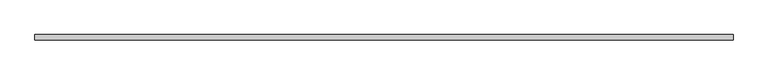
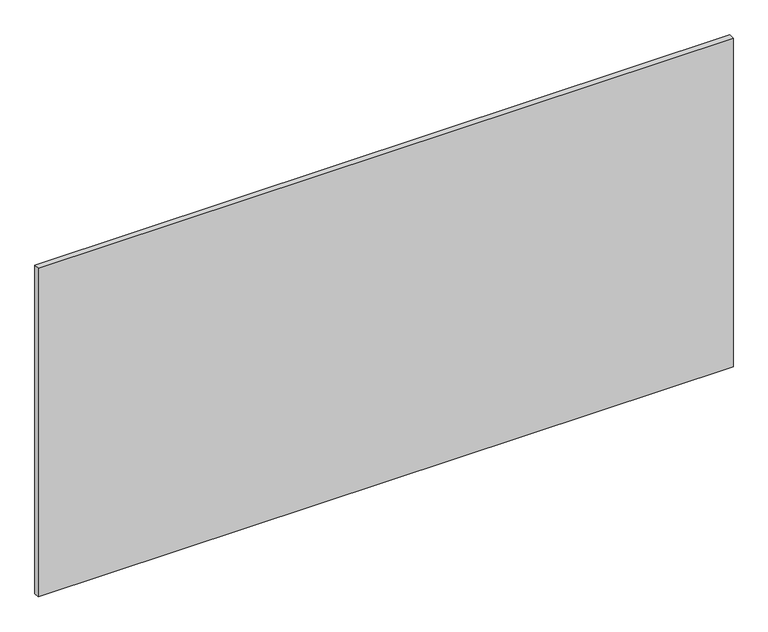
"""IFC4 building model written with IfcOpenShell, lengths in millimetres: proxy geometry, Inner panel:Inner panel:1:Inner panel:1 : Inner panel:Inner panel:300324:300043:Inner panel:1:Inner panel:1 : Inner panel:Inner panel:300324:300043 : Inner panel:Inner panel:1:Inner panel:1 : Inner panel:Inner panel:300324:300043:21 : Inner panel:Inner panel:1:Inner panel:1 : Inner panel:Inner panel:300324:300043:Inner panel:1:Inner panel:1 : Inner panel:Inner panel:300324:300043 : Inner panel:Inner panel:1:Inner panel:1 : Inner panel:Inner panel:300324:300043:300031."""

from ifc_helpers import new_model, si_unit, frame, origin, place, context, project, spatial, polyline, outline, extrude, source, transform, mapped, element, save


def generic_models_ae8239df(model_context):
    return source(origin(), model_context, "Body", "SweptSolid", [
        extrude(outline(polyline([(590067.7867239, -568186.6413841), (592506.1867239, -568186.6413841), (592506.1867239, -568205.6913841), (590067.7867239, -568205.6913841), (590067.7867239, -568186.6413841)])), frame((0.0, 0.0, 3721.1), z_axis=(0.0, 0.0, 1.0), x_axis=(1.0, 0.0, 0.0)), (0.0, 0.0, 1.0), 1219.2),
    ])


if __name__ == "__main__":
    model = new_model("IFC4")
    model_context = context("Model", 3, world=origin())
    ifc_project = project(units=[si_unit("LENGTHUNIT", "METRE", prefix="MILLI")], contexts=[model_context])
    site = spatial("IfcSite", under=ifc_project)
    building = spatial("IfcBuilding", under=site)
    placement = place(None, origin())
    generic_models_shape = generic_models_ae8239df(model_context)
    element("IfcBuildingElementProxy", 1, Name="Inner panel:Inner panel:1:Inner panel:1 : Inner panel:Inner panel:300324:300043:Inner panel:1:Inner panel:1 : Inner panel:Inner panel:300324:300043 : Inner panel:Inner panel:1:Inner panel:1 : Inner panel:Inner panel:300324:300043:21 : Inner panel:Inner panel:1:Inner panel:1 : Inner panel:Inner panel:300324:300043:Inner panel:1:Inner panel:1 : Inner panel:Inner panel:300324:300043 : Inner panel:Inner panel:1:Inner panel:1 : Inner panel:Inner panel:300324:300043:300031", ObjectType="Inner panel:Inner panel:1:Inner panel:1 : Inner panel:Inner panel:300324:300043:Inner panel:1:Inner panel:1 : Inner panel:Inner panel:300324:300043 : Inner panel:Inner panel:1:Inner panel:1 : Inner panel:Inner panel:300324:300043:21 : Inner panel:Inner panel:1:Inner panel:1 : Inner panel:Inner panel:300324:300043:Inner panel:1:Inner panel:1 : Inner panel:Inner panel:300324:300043 : Inner panel:Inner panel:1:Inner panel:1 : Inner panel:Inner panel:300324:300043:300031", at=placement, inside=building, context=model_context, shape_type="MappedRepresentation", body=[
        mapped(generic_models_shape, transform((0.0, 0.0, 0.0), x_axis=(1.0, 0.0, 0.0), y_axis=(0.0, 1.0, 0.0), z_axis=(0.0, 0.0, 1.0))),
    ])
    save(model, "model.ifc")

# Revit data of these elements
# Type "Inner panel:Inner panel:1:Inner panel:1 : Inner panel:Inner panel:300324:300043:Inner panel:1:Inner panel:1 : Inner panel:Inner panel:300324:300043 : Inner panel:Inner panel:1:Inner panel:1 : Inner panel:Inner panel:300324:300043:21 : Inner panel:Inner panel:1:Inner panel:1 : Inner panel:Inner panel:300324:300043:Inner panel:1:Inner panel:1 : Inner panel:Inner panel:300324:300043 : Inner panel:Inner panel:1:Inner panel:1 : Inner panel:Inner panel:300324:300043:300031"
#   NameOverride = "Inner panel:Inner panel:1:Inner panel:1 : Inner panel:Inner panel:300324:300043:Inner panel:1:Inner panel:1 : Inner panel:Inner panel:300324:300043 : Inner panel:Inner panel:1:Inner panel:1 : Inner panel:Inner panel:300324:300043:300031"
#   ObjectTypeOverride = "Inner panel:1:Inner panel:1 : Inner panel:Inner panel:300324:300043 : Inner panel:Inner panel:1:Inner panel:1 : Inner panel:Inner panel:300324:300043"
#   Reference = "Inner panel"
#   Tag = "300031"
# Element 1 (IfcBuildingElementProxy, "Inner panel:Inner panel:1:Inner panel:1 : Inner panel:Inner panel:300324:300043:Inner panel:1:Inner panel:1 : Inner panel:Inner panel:300324:300043 : Inner panel:Inner panel:1:Inner panel:1 : Inner panel:Inner panel:300324:300043:21 : Inner panel:Inner panel:1:Inner panel:1 : Inner panel:Inner panel:300324:300043:Inner panel:1:Inner panel:1 : Inner panel:Inner panel:300324:300043 : Inner panel:Inner panel:1:Inner panel:1 : Inner panel:Inner panel:300324:300043:300031")
#   Materials on its faces: "3/4\" PREFINISHED STAINED/SEALED PLYWOOD (FINISH: GRADE B,  FLAME SPREAD: CLASS B)"
# Materials
#   "3/4\" PREFINISHED STAINED/SEALED PLYWOOD (FINISH: GRADE B,  FLAME SPREAD: CLASS B)": class "Wood", colour RGB 149 120 74, transparency 0, Description = "Plywood, sheathing grade", Cost = 0
